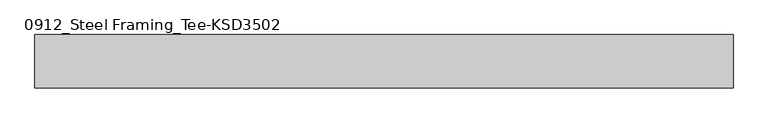
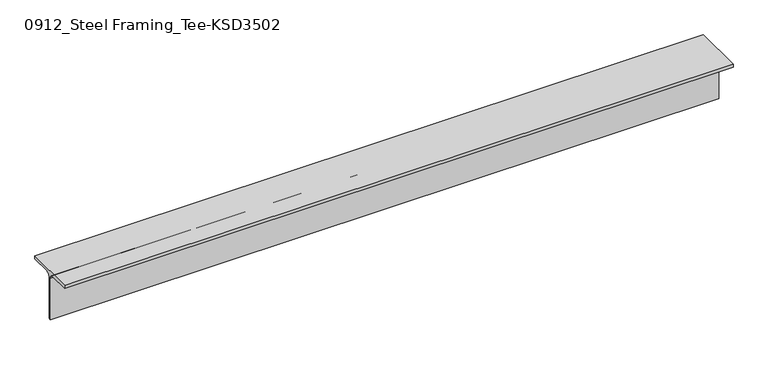
"""IFC4 building model written with IfcOpenShell, lengths in millimetres: member geometry, 0912_Steel Framing_Tee-KSD3502 : H_SB_ASB_CT-150x150x6.5x9."""

from ifc_helpers import new_model, si_unit, point, frame, frame_2d, origin, place, context, project, spatial, polyline, circle_curve, trimmed, segment, composite_curve, outline, extrude, source, transform, mapped, element, save


def member_0912_steel_framing_tee_ksd3502_3dd86a91(model_context):
    return source(origin(), model_context, "Body", "SweptSolid", [
        extrude(outline(composite_curve([segment(polyline([(75.0, 75.0), (75.0, 66.0), (16.25, 66.0)]), True, "CONTINUOUS"), segment(trimmed(circle_curve(frame_2d((16.25, 53.0)), 13.0), [point((16.25, 66.0))], [point((3.25, 53.0))], True, "CARTESIAN"), True, "CONTINUOUS"), segment(polyline([(3.25, 53.0), (3.25, -75.0), (-3.25, -75.0), (-3.25, 53.0)]), True, "CONTINUOUS"), segment(trimmed(circle_curve(frame_2d((-16.25, 53.0)), 13.0), [point((-3.25, 53.0))], [point((-16.25, 66.0))], True, "CARTESIAN"), True, "CONTINUOUS"), segment(polyline([(-16.25, 66.0), (-75.0, 66.0), (-75.0, 75.0), (75.0, 75.0)]), True, "CONTINUOUS")], self_intersect=False)), frame((-1113.65, 0.0, 0.0), z_axis=(1.0, 0.0, 0.0), x_axis=(0.0, 1.0, 0.0)), (0.0, 0.0, 1.0), 1955.9),
    ])


if __name__ == "__main__":
    model = new_model("IFC4")
    model_context = context("Model", 3, world=origin())
    ifc_project = project(units=[si_unit("LENGTHUNIT", "METRE", prefix="MILLI")], contexts=[model_context])
    site = spatial("IfcSite", under=ifc_project)
    building = spatial("IfcBuilding", under=site)
    placement = place(None, origin())
    member_0912_steel_framing_tee_ksd3502_shape = member_0912_steel_framing_tee_ksd3502_3dd86a91(model_context)
    element("IfcMember", 1, ObjectType="0912_Steel Framing_Tee-KSD3502 : H_SB_ASB_CT-150x150x6.5x9", at=placement, inside=building, context=model_context, shape_type="MappedRepresentation", body=[
        mapped(member_0912_steel_framing_tee_ksd3502_shape, transform((0.0, 0.0, 0.0), x_axis=(1.0, 0.0, 0.0), y_axis=(0.0, 1.0, 0.0), z_axis=(0.0, 0.0, 1.0))),
    ])
    save(model, "model.ifc")

# Revit data of these elements
# Type "0912_Steel Framing_Tee-KSD3502 : H_SB_ASB_CT-150x150x6.5x9"
#   H_WM Code_1 = "S01AA003-00001 | Main Steel Structure Fabrication Work | Shelter/Building | Light Steel - Standard (30KG/M>Weight) | Material: (   )"
#   H_WM Code_2 = "S03AA029-00001 | Main Steel Structure Erection Work | Shelter/Building | Light Steel (30KG/M>Weight) | Material: (   )"
#   H_WM Code_3 = "S01AA010-00001 | Main Steel Structure Fabrication Work | Shelter/Building | Steel Painting/Coating | for Non-Fireproofed Steel Surface, Surface Preparation, Primer, Second & Final Coat | Material: (   )"
#   H_Q'ty Cal Type Tag = "SB-Q2"
#   Width = 15.0 cm
#   Web Thickness = 0.65 cm
#   Web Fillet = 1.3 cm
#   Section Area = 23.39 cm²
#   Perimeter = 0.60 m²/m
#   Nominal Weight = 18.40 kgf/m
#   Height = 15.0 cm
#   Flange Thickness = 0.9 cm
#   Centroid Vertical = 7.5 cm
#   Centroid Horizontal = 7.5 cm
#   Length [instance default] = 1.5000 m
#   Structural Material [instance default] = Steel, 45-345
#   Warping Constant = (empty or 0)
#   Torsional Moment of Inertia = 0
#   Section Name Key = ""
#   Plastic Modulus weak axis = 0
#   Plastic Modulus strong axis = 0
#   Moment of Inertia weak axis = 0
#   Moment of Inertia strong axis = 0
#   Elastic Modulus weak axis = 0
#   Elastic Modulus strong axis = 0
#   Bolt Spacing = 0
#   Assembly Code = ""
# Element 1 (IfcMember, "0912_Steel Framing_Tee-KSD3502 : H_SB_ASB_CT-150x150x6.5x9")
#   Structural Material = none
# Materials
#   "Steel, 45-345": class "Metal", colour RGB 189 187 185, transparency 0, Description = "Steel 345 MPa", Cost = 0
